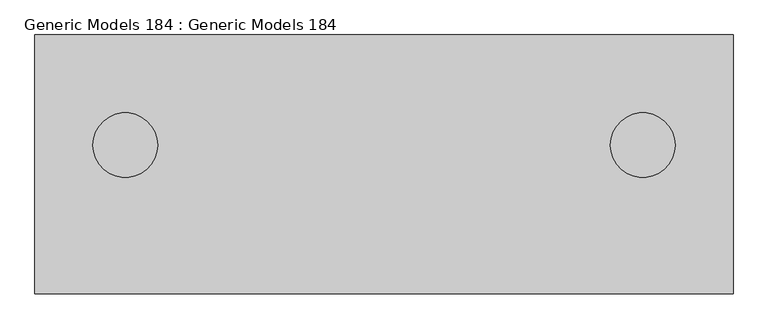
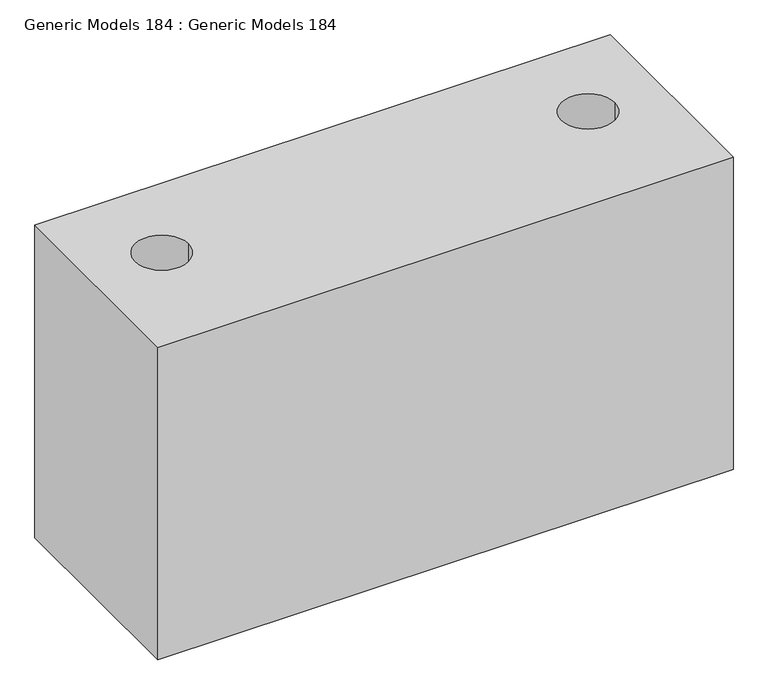
"""IFC4 building model written with IfcOpenShell, lengths in millimetres: proxy geometry, Generic Models 184 : Generic Models 184."""

from ifc_helpers import new_model, si_unit, frame, origin, place, context, project, spatial, polyline, circle_curve, source, transform, mapped, element, save
from ifc_brep_helpers import plane_surface, revolved_surface, advanced_brep


def generic_models_184_generic_models_184_067f22a4(model_context):
    return source(origin(), model_context, "Body", "AdvancedBrep", [
        advanced_brep(
        [(57021.4125, 977.9, -23.9117188), (53732.1125, 977.9, -23.9117188), (53732.1125, -241.3, -23.9117188), (57021.4125, -241.3, -23.9117188), (56443.5625, 458.7875, -23.9117188), (56748.3625, 458.7875, -23.9117188), (54005.1625, 458.7875, -23.9117188), (54309.9625, 458.7875, -23.9117188), (57021.4125, 977.9, -1915.3720904), (57021.4125, -241.3, -1915.3720904), (53732.1125, -241.3, -1915.3720904), (53732.1125, 977.9, -1915.3720904), (56443.5625, 458.7875, -1219.2), (56748.3625, 458.7875, -1219.2), (54005.1625, 458.7875, -1219.2), (54309.9625, 458.7875, -1219.2)],
        [
            (0, 1),
            (1, 2),
            (2, 3),
            (3, 0),
            (4, 5, circle_curve(frame((56595.9625, 458.7875, -23.9117188), z_axis=(0.0, 0.0, -1.0), x_axis=(1.0, 0.0, 0.0)), 152.4)),
            (5, 4, circle_curve(frame((56595.9625, 458.7875, -23.9117188), z_axis=(0.0, 0.0, -1.0), x_axis=(1.0, 0.0, 0.0)), 152.4)),
            (6, 7, circle_curve(frame((54157.5625, 458.7875, -23.9117188), z_axis=(0.0, 0.0, -1.0), x_axis=(1.0, 0.0, 0.0)), 152.4)),
            (7, 6, circle_curve(frame((54157.5625, 458.7875, -23.9117188), z_axis=(0.0, 0.0, -1.0), x_axis=(1.0, 0.0, 0.0)), 152.4)),
            (8, 9),
            (9, 10),
            (10, 11),
            (11, 8),
            (0, 8),
            (11, 1),
            (10, 2),
            (9, 3),
            (12, 13, circle_curve(frame((56595.9625, 458.7875, -1219.2), z_axis=(0.0, 0.0, 1.0), x_axis=(1.0, 0.0, 0.0)), 152.4)),
            (13, 12, circle_curve(frame((56595.9625, 458.7875, -1219.2), z_axis=(0.0, 0.0, 1.0), x_axis=(1.0, 0.0, 0.0)), 152.4)),
            (14, 15, circle_curve(frame((54157.5625, 458.7875, -1219.2), z_axis=(0.0, 0.0, 1.0), x_axis=(1.0, 0.0, 0.0)), 152.4)),
            (15, 14, circle_curve(frame((54157.5625, 458.7875, -1219.2), z_axis=(0.0, 0.0, 1.0), x_axis=(1.0, 0.0, 0.0)), 152.4)),
            (13, 5),
            (4, 12),
            (15, 7),
            (6, 14),
        ],
        [
            plane_surface(frame((53732.1125, 977.9, -23.9117188), z_axis=(0.0, 0.0, 1.0), x_axis=(-1.0, 0.0, 0.0))),
            plane_surface(frame((53732.1125, 977.9, -1915.3720904), z_axis=(0.0, 0.0, -1.0), x_axis=(1.0, 0.0, 0.0))),
            plane_surface(frame((57021.4125, 977.9, -23.9117188), z_axis=(0.0, 1.0, 0.0), x_axis=(0.0, 0.0, -1.0))),
            plane_surface(frame((53732.1125, 977.9, -23.9117188), z_axis=(-1.0, 0.0, 0.0), x_axis=(0.0, 0.0, -1.0))),
            plane_surface(frame((53732.1125, -241.3, -23.9117188), z_axis=(0.0, -1.0, 0.0), x_axis=(0.0, 0.0, -1.0))),
            plane_surface(frame((57021.4125, -241.3, -23.9117188), z_axis=(1.0, 0.0, 0.0), x_axis=(0.0, 0.0, -1.0))),
            plane_surface(frame((56748.3625, 458.7875, -1219.2), z_axis=(0.0, 0.0, 1.0), x_axis=(0.0, -1.0, 0.0))),
            revolved_surface(polyline([(56748.3625, 458.7875, -23.911718800000017), (56748.3625, 458.7875, -1219.2)]), (56595.9625, 458.7875, -1219.2), (0.0, 0.0, 1.0)),
            revolved_surface(polyline([(54309.9625, 458.7875, -23.9117188), (54309.9625, 458.7875, -1219.2)]), (54157.5625, 458.7875, 0.0), (0.0, 0.0, 1.0)),
        ],
        [
            (0, [[1, 2, 3, 4], [5, 6], [7, 8]]),
            (1, [[9, 10, 11, 12]]),
            (2, [[-1, 13, -12, 14]]),
            (3, [[-2, -14, -11, 15]]),
            (4, [[-3, -15, -10, 16]]),
            (5, [[-4, -16, -9, -13]]),
            (6, [[17, 18]]),
            (6, [[19, 20]]),
            (7, [[-18, 21, -5, 22]]),
            (7, [[-17, -22, -6, -21]]),
            (8, [[-20, 23, -7, 24]]),
            (8, [[-19, -24, -8, -23]]),
        ],
    ),
    ])


if __name__ == "__main__":
    model = new_model("IFC4")
    model_context = context("Model", 3, world=origin())
    ifc_project = project(units=[si_unit("LENGTHUNIT", "METRE", prefix="MILLI")], contexts=[model_context])
    site = spatial("IfcSite", under=ifc_project)
    building = spatial("IfcBuilding", under=site)
    placement = place(None, origin())
    generic_models_184_generic_models_184_shape = generic_models_184_generic_models_184_067f22a4(model_context)
    element("IfcBuildingElementProxy", 1, Name="Generic Models 184 : Generic Models 184", ObjectType="Generic Models 184 : Generic Models 184", at=placement, inside=building, context=model_context, shape_type="MappedRepresentation", body=[
        mapped(generic_models_184_generic_models_184_shape, transform((0.0, 0.0, 0.0), x_axis=(1.0, 0.0, 0.0), y_axis=(0.0, 1.0, 0.0), z_axis=(0.0, 0.0, 1.0))),
    ])
    save(model, "model.ifc")

# Revit data of these elements
# Element 1 (IfcBuildingElementProxy, "Generic Models 184 : Generic Models 184")
#   Materials on its faces: "GRADE"
# Materials
#   "GRADE": class "Generic", colour RGB 255 255 255, transparency 0, Description = "Soil", Cost = 0
